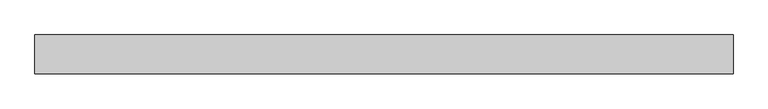
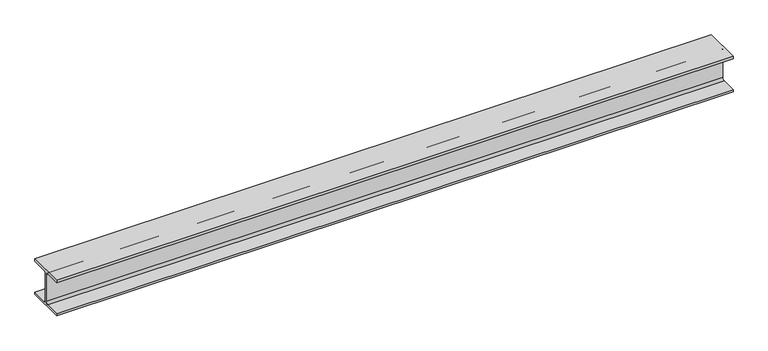
"""IFC4 building model written with IfcOpenShell, lengths in millimetres: beam geometry, 0912_Steel Framing_H-KSD3502 : H_SB_ASB_H-200x200x8x12."""

from ifc_helpers import new_model, si_unit, point, frame, frame_2d, origin, place, context, project, spatial, polyline, circle_curve, trimmed, segment, composite_curve, outline, extrude, source, transform, mapped, element, save


def beam_c0af7261(model_context):
    return source(origin(), model_context, "Body", "SweptSolid", [
        extrude(outline(composite_curve([segment(polyline([(100.0, -88.0), (100.0, -100.0), (-100.0, -100.0), (-100.0, -88.0), (-17.0, -88.0)]), True, "CONTINUOUS"), segment(trimmed(circle_curve(frame_2d((-17.0, -75.0)), 13.0), [point((-17.0, -88.0))], [point((-4.0, -75.0))], True, "CARTESIAN"), True, "CONTINUOUS"), segment(polyline([(-4.0, -75.0), (-4.0, 75.0)]), True, "CONTINUOUS"), segment(trimmed(circle_curve(frame_2d((-17.0, 75.0)), 13.0), [point((-4.0, 75.0))], [point((-17.0, 88.0))], True, "CARTESIAN"), True, "CONTINUOUS"), segment(polyline([(-17.0, 88.0), (-100.0, 88.0), (-100.0, 100.0), (100.0, 100.0), (100.0, 88.0), (17.0, 88.0)]), True, "CONTINUOUS"), segment(trimmed(circle_curve(frame_2d((17.0, 75.0)), 13.0), [point((17.0, 88.0))], [point((4.0, 75.0))], True, "CARTESIAN"), True, "CONTINUOUS"), segment(polyline([(4.0, 75.0), (4.0, -75.0)]), True, "CONTINUOUS"), segment(trimmed(circle_curve(frame_2d((17.0, -75.0)), 13.0), [point((4.0, -75.0))], [point((17.0, -88.0))], True, "CARTESIAN"), True, "CONTINUOUS"), segment(polyline([(17.0, -88.0), (100.0, -88.0)]), True, "CONTINUOUS")], self_intersect=False)), frame((-1668.0611839, 0.0, 0.0), z_axis=(1.0, 0.0, 0.0), x_axis=(0.0, 1.0, 0.0)), (0.0, 0.0, 1.0), 3604.1166019),
    ])


if __name__ == "__main__":
    model = new_model("IFC4")
    model_context = context("Model", 3, world=origin())
    ifc_project = project(units=[si_unit("LENGTHUNIT", "METRE", prefix="MILLI")], contexts=[model_context])
    site = spatial("IfcSite", under=ifc_project)
    building = spatial("IfcBuilding", under=site)
    placement = place(None, origin())
    beam_shape = beam_c0af7261(model_context)
    element("IfcBeam", 1, ObjectType="0912_Steel Framing_H-KSD3502 : H_SB_ASB_H-200x200x8x12", at=placement, inside=building, context=model_context, shape_type="MappedRepresentation", body=[
        mapped(beam_shape, transform((0.0, 0.0, 0.0), x_axis=(1.0, 0.0, 0.0), y_axis=(0.0, 1.0, 0.0), z_axis=(0.0, 0.0, 1.0))),
    ])
    save(model, "model.ifc")

# Revit data of these elements
# Type "0912_Steel Framing_H-KSD3502 : H_SB_ASB_H-200x200x8x12"
#   H_WM Code_1 = "S01AA002-00001 | Main Steel Structure Fabrication Work | Shelter/Building | Medium Steel - Standard (90KG/M>Weight≥30KG/M) | Material: (   )"
#   H_WM Code_2 = "S03AA028-00001 | Main Steel Structure Erection Work | Shelter/Building | Medium Steel (90KG/M>Weight≥30KG/M) | Material: (   )"
#   H_WM Code_3 = "S01AA010-00001 | Main Steel Structure Fabrication Work | Shelter/Building | Steel Painting/Coating | for Non-Fireproofed Steel Surface, Surface Preparation, Primer, Second & Final Coat | Material: (   )"
#   H_Q'ty Cal Type Tag = "SB-Q2"
#   Width = 20.0 cm
#   Web Thickness = 0.8 cm
#   Web Fillet = 1.3 cm
#   Warping Constant = 141000.0 cm⁶
#   W = 0
#   Torsional Moment of Inertia = 26.2485 cm⁴
#   Section Area = 63.53 cm²
#   Plastic Modulus weak axis = 244.0 cm³
#   Plastic Modulus strong axis = 525.0 cm³
#   Perimeter = 1.16 m²/m
#   Nominal Weight = 49.90 kgf/m
#   Moment of Inertia weak axis = 1600.00 cm⁴
#   Moment of Inertia strong axis = 4720.00 cm⁴
#   Height = 20.0 cm
#   Flange Thickness = 1.2 cm
#   Elastic Modulus weak axis = 160.0 cm³
#   Elastic Modulus strong axis = 472.0 cm³
#   Centroid Vertical = 10.0 cm
#   Centroid Horizontal = 10.0 cm
#   Ix = 47200000
#   Length [instance default] = 1.5240 m
#   Zx = 525000
#   b = 0.2000 m
#   h = 0.2000 m
#   r = 0.0130 m
#   s = 0.0080 m
#   t = 0.0120 m
#   A = 0.006353 m²
#   Structural Material [instance default] = Steel, 45-345
#   Assembly Code = ""
# Element 1 (IfcBeam, "0912_Steel Framing_H-KSD3502 : H_SB_ASB_H-200x200x8x12")
#   Structural Material = none
# Materials
#   "Steel, 45-345": class "Metal", colour RGB 189 187 185, transparency 0, Description = "Steel 345 MPa", Cost = 0
